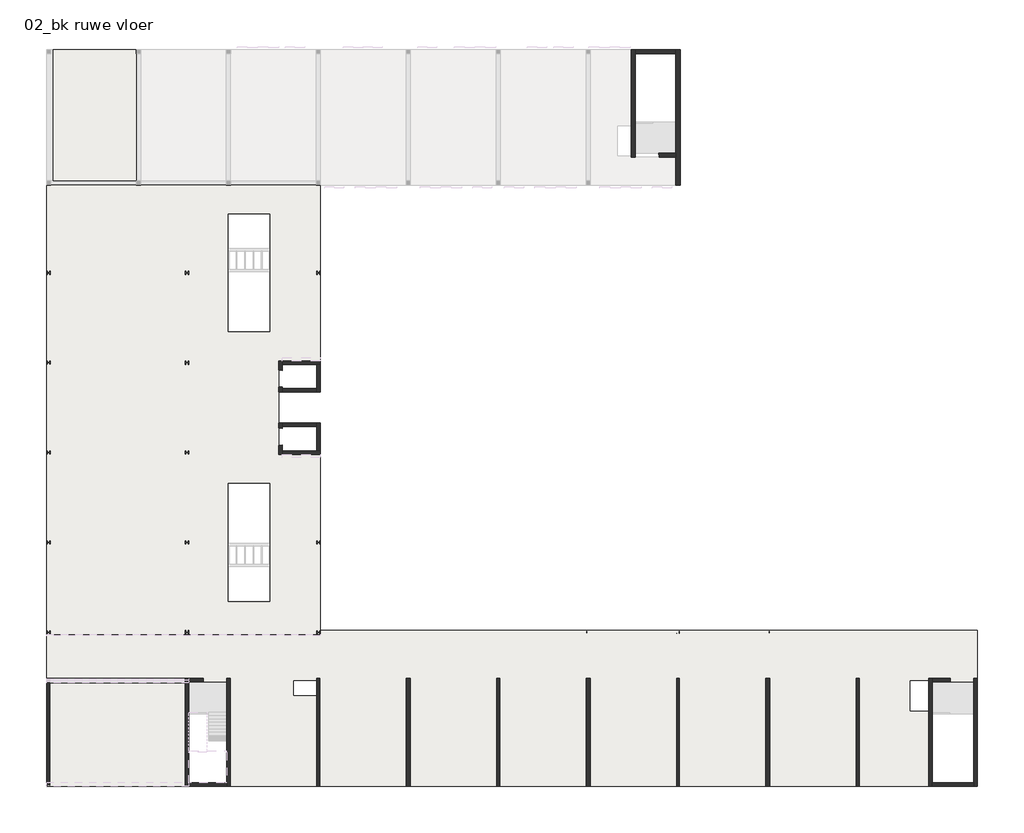
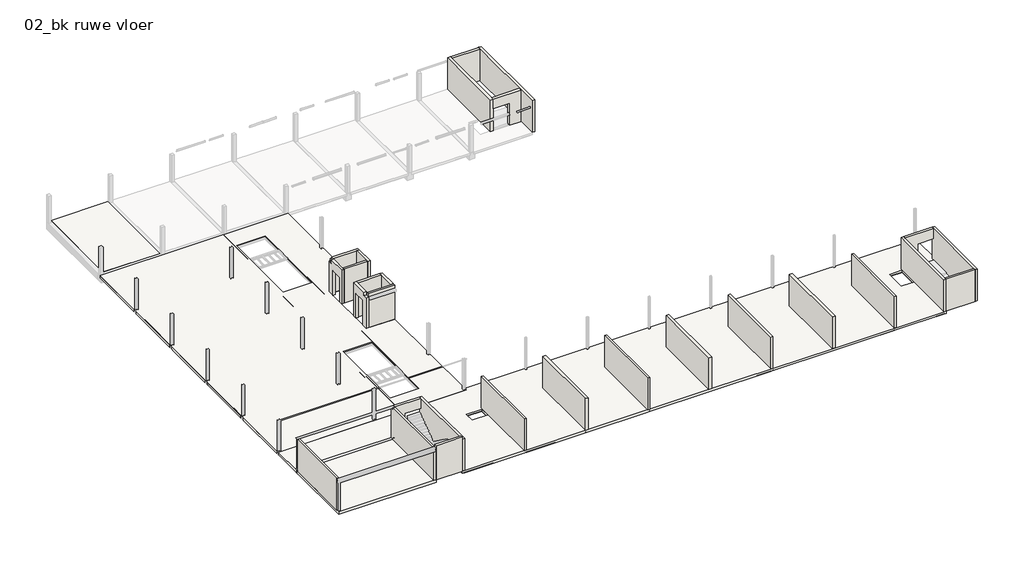
# One storey, part 1 of 3: 28 walls, 20 slabs.
# Revit data of these elements (continued)
# Element 16 (IfcSlab, "NLRS_23_FL_kanaalplaat 260_gen_rsf") (continued)
#   IfcGUID = "13lTCcCQ95UOWcvnmPh7yS"
#   built-in parameter 1001955 = 1.5708 (stored number, unit not read)
#   Height Offset From Level = -70 mm
#   built-in parameter 1001954 = 1
#   IsExternal = no
#   LoadBearing = yes
#   Phase Created = NLRS_nieuw
#   Materials on its faces: "NLRS_f2_beton prefab_gen_rsf"
# Element 17 (IfcSlab, "NLRS_23_FL_breedplaat 260_gen_rsf")
#   IfcGUID = "3aMdMHoe12P9KDGPyaIhfl"
#   built-in parameter 1001955 = 1.5708 (stored number, unit not read)
#   Height Offset From Level = 0 mm
#   built-in parameter 1001954 = 1
#   IsExternal = no
#   LoadBearing = yes
#   Phase Created = NLRS_nieuw
#   Materials on its faces: "NLRS_f2_beton ihwg_gen_rsf"
# Element 18 (IfcSlab, "NLRS_23_FL_breedplaat schil 60_gen_rsf")
#   IfcGUID = "30fJl_yZvFzewSfsmFGxtY"
#   Comments = ""
#   Height Offset From Level = -200 mm
#   built-in parameter 1001954 = 1
#   IsExternal = no
#   LoadBearing = yes
#   Phase Created = NLRS_nieuw
#   Materials on its faces: "NLRS_f2_beton prefab_gen_rsf"
# Element 19 (IfcSlab, "NLRS_23_FL_breedplaat schil 60_gen_rsf")
#   IfcGUID = "2NjBJrSTnArAq_EA_3B3B5"
#   Comments = ""
#   built-in parameter 1001955 = -1.5708 (stored number, unit not read)
#   Height Offset From Level = -200 mm
#   built-in parameter 1001954 = 1
#   IsExternal = no
#   LoadBearing = yes
#   Phase Created = NLRS_nieuw
#   Materials on its faces: "NLRS_f2_beton prefab_gen_rsf"
# Element 20 (IfcSlab, "NLRS_23_FL_breedplaat schil 60_gen_rsf")
#   IfcGUID = "2qE$kEBNbDT8O3EB3ypEdt"
#   Comments = ""
#   Height Offset From Level = -200 mm
#   built-in parameter 1001954 = 1
#   IsExternal = no
#   LoadBearing = yes
#   Phase Created = NLRS_nieuw
#   Materials on its faces: "NLRS_f2_beton prefab_gen_rsf"
# Element 21 (IfcWall, "NLRS_22_WA_beton ihw 250_gen_rsf")
#   IfcGUID = "13lTCcCQ95UOWcvnmPh77b"
#   Comments = ""
#   Top Offset = 0 mm
#   Base Offset = 0 mm
#   wall height = 3540 mm
#   IsExternal = no
#   LoadBearing = yes
#   Phase Created = NLRS_nieuw
#   Base Constraint = 02_bk ruwe vloer
#   Top Constraint = 03_ok ruwe vloer
#   Materials on its faces: "NLRS_f2_beton ihwg_gen_rsf"
# Element 22 (IfcWall, "NLRS_22_WA_beton ihw 250_gen_rsf")
#   IfcGUID = "13lTCcCQ95UOWcvnmPh77d"
#   Comments = ""
#   Top Offset = 0 mm
#   Base Offset = 0 mm
#   wall height = 3540 mm
#   IsExternal = no
#   LoadBearing = yes
#   Phase Created = NLRS_nieuw
#   Base Constraint = 02_bk ruwe vloer
#   Top Constraint = 03_ok ruwe vloer
#   Materials on its faces: "NLRS_f2_beton ihwg_gen_rsf"
# Element 23 (IfcWall, "NLRS_22_WA_kalkzandsteen CS12 214_gen_rsf")
#   IfcGUID = "13lTCcCQ95UOWcvnmPh77X"
#   Comments = ""
#   Top Offset = 0 mm
#   Base Offset = 0 mm
#   wall height = 3540 mm
#   IsExternal = no
#   LoadBearing = yes
#   Phase Created = NLRS_nieuw
#   Base Constraint = 02_bk ruwe vloer
#   Top Constraint = 03_ok ruwe vloer
#   Materials on its faces: "NLRS_f1_kalkzandsteen_gen_rsf"
# Element 24 (IfcWall, "NLRS_22_WA_beton ihw 300_gen_rsf")
#   IfcGUID = "13lTCcCQ95UOWcvnmPh77Z"
#   Comments = ""
#   Top Offset = 0 mm
#   Base Offset = 0 mm
#   wall height = 3540 mm
#   IsExternal = no
#   LoadBearing = yes
#   Phase Created = NLRS_nieuw
#   Base Constraint = 02_bk ruwe vloer
#   Top Constraint = 03_ok ruwe vloer
#   Materials on its faces: "NLRS_f2_beton ihwg_gen_rsf"
# Element 25 (IfcWall, "NLRS_22_WA_kalkzandsteen CS12 214_gen_rsf")
#   IfcGUID = "13lTCcCQ95UOWcvnmPh78T"
#   Comments = ""
#   Top Offset = 0 mm
#   Base Offset = 0 mm
#   wall height = 3540 mm
#   IsExternal = no
#   LoadBearing = yes
#   Phase Created = NLRS_nieuw
#   Base Constraint = 02_bk ruwe vloer
#   Top Constraint = 03_ok ruwe vloer
#   Materials on its faces: "NLRS_f1_kalkzandsteen_gen_rsf"
# Element 26 (IfcWall, "NLRS_22_WA_beton ihw 300_gen_rsf")
#   IfcGUID = "13lTCcCQ95UOWcvnmPh78V"
#   Comments = ""
#   Top Offset = 0 mm
#   Base Offset = 0 mm
#   wall height = 3540 mm
#   IsExternal = no
#   LoadBearing = yes
#   Phase Created = NLRS_nieuw
#   Base Constraint = 02_bk ruwe vloer
#   Top Constraint = 03_ok ruwe vloer
#   Materials on its faces: "NLRS_f2_beton ihwg_gen_rsf"
# Element 27 (IfcWall, "NLRS_22_WA_kalkzandsteen CS12 214_gen_rsf")
#   IfcGUID = "13lTCcCQ95UOWcvnmPh78P"
#   Comments = ""
#   Top Offset = 0 mm
#   Base Offset = 0 mm
#   wall height = 3540 mm
#   IsExternal = no
#   LoadBearing = yes
#   Phase Created = NLRS_nieuw
#   Base Constraint = 02_bk ruwe vloer
#   Top Constraint = 03_ok ruwe vloer
#   Materials on its faces: "NLRS_f1_kalkzandsteen_gen_rsf"
# Element 28 (IfcWall, "NLRS_22_WA_beton ihw 300_gen_rsf")
#   IfcGUID = "13lTCcCQ95UOWcvnmPh78R"
#   Comments = ""
#   Top Offset = 0 mm
#   Base Offset = 0 mm
#   wall height = 3540 mm
#   IsExternal = no
#   LoadBearing = yes
#   Phase Created = NLRS_nieuw
#   Base Constraint = 02_bk ruwe vloer
#   Top Constraint = 03_ok ruwe vloer
#   Materials on its faces: "NLRS_f2_beton ihwg_gen_rsf"
# Element 29 (IfcWall, "NLRS_22_WA_kalkzandsteen CS12 214_gen_rsf")
#   IfcGUID = "13lTCcCQ95UOWcvnmPh78L"
#   Comments = ""
#   Top Offset = 0 mm
#   Base Offset = 0 mm
#   wall height = 3540 mm
#   IsExternal = no
#   LoadBearing = yes
#   Phase Created = NLRS_nieuw
#   Base Constraint = 02_bk ruwe vloer
#   Top Constraint = 03_ok ruwe vloer
#   Materials on its faces: "NLRS_f1_kalkzandsteen_gen_rsf"
# Element 30 (IfcWall, "NLRS_21_WA_beton ihw 250_gen_rsf")
#   IfcGUID = "13lTCcCQ95UOWcvnmPh78N"
#   Comments = ""
#   Top Offset = 0 mm
#   Base Offset = 0 mm
#   wall height = 3540 mm
#   IsExternal = yes
#   LoadBearing = yes
#   Phase Created = NLRS_nieuw
#   Base Constraint = 02_bk ruwe vloer
#   Top Constraint = 03_ok ruwe vloer
#   Materials on its faces: "NLRS_f2_beton ihwg_gen_rsf"
# Element 31 (IfcWall, "NLRS_21_WA_kalkzandsteen CS12 214_gen_rsf")
#   IfcGUID = "13lTCcCQ95UOWcvnmPh78H"
#   Comments = ""
#   Top Offset = 0 mm
#   Base Offset = 0 mm
#   wall height = 3540 mm
#   IsExternal = yes
#   LoadBearing = yes
#   Phase Created = NLRS_nieuw
#   Base Constraint = 02_bk ruwe vloer
#   Top Constraint = 03_ok ruwe vloer
#   Materials on its faces: "NLRS_f1_kalkzandsteen_gen_rsf"
# Element 32 (IfcWall, "NLRS_21_WA_beton ihw 250_gen_rsf")
#   IfcGUID = "13lTCcCQ95UOWcvnmPh78J"
#   Top Offset = 0 mm
#   Base Offset = 0 mm
#   wall height = 3800 mm
#   IsExternal = yes
#   LoadBearing = yes
#   Phase Created = NLRS_nieuw
#   Base Constraint = 02_bk ruwe vloer
#   Top Constraint = 03_bk. ruwe vloer
#   Materials on its faces: "NLRS_f2_beton ihwg_gen_rsf"
# Element 33 (IfcWall, "NLRS_22_WA_beton ihw 250_gen_rsf")
#   IfcGUID = "13lTCcCQ95UOWcvnmPh78D"
#   Top Offset = 0 mm
#   Base Offset = 0 mm
#   wall height = 3540 mm
#   IsExternal = no
#   LoadBearing = yes
#   Phase Created = NLRS_nieuw
#   Base Constraint = 02_bk ruwe vloer
#   Top Constraint = 03_ok ruwe vloer
#   Materials on its faces: "NLRS_f2_beton ihwg_gen_rsf"
# Element 34 (IfcWall, "NLRS_22_WA_beton ihw 250_gen_rsf")
#   IfcGUID = "13lTCcCQ95UOWcvnmPh78F"
#   Comments = ""
#   Top Offset = 0 mm
#   Base Offset = 0 mm
#   wall height = 3540 mm
#   IsExternal = no
#   LoadBearing = yes
#   Phase Created = NLRS_nieuw
#   Base Constraint = 02_bk ruwe vloer
#   Top Constraint = 03_ok ruwe vloer
#   Materials on its faces: "NLRS_f2_beton ihwg_gen_rsf"
# Element 35 (IfcWall, "NLRS_21_WA_beton ihw 250_gen_rsf")
#   IfcGUID = "13lTCcCQ95UOWcvnmPh789"
#   Top Offset = 0 mm
#   Base Offset = 0 mm
#   wall height = 3540 mm
#   IsExternal = yes
#   LoadBearing = yes
#   Phase Created = NLRS_nieuw
#   Base Constraint = 02_bk ruwe vloer
#   Top Constraint = 03_ok ruwe vloer
#   Materials on its faces: "NLRS_f2_beton ihwg_gen_rsf"
# Element 36 (IfcWall, "NLRS_22_WA_beton ihw 250_gen_rsf")
#   IfcGUID = "13lTCcCQ95UOWcvnmPh78B"
#   Top Offset = 0 mm
#   Base Offset = 0 mm
#   wall height = 3540 mm
#   IsExternal = no
#   LoadBearing = yes
#   Phase Created = NLRS_nieuw
#   Base Constraint = 02_bk ruwe vloer
#   Top Constraint = 03_ok ruwe vloer
#   Materials on its faces: "NLRS_f2_beton ihwg_gen_rsf"
# Element 37 (IfcWall, "NLRS_22_WA_beton prefab 300_gen_rsf")
#   IfcGUID = "13lTCcCQ95UOWcvnmPh79n"
#   Comments = ""
#   built-in parameter 1001111 = 20 mm
#   Top Offset = 0 mm
#   Base Offset = 20 mm
#   wall height = 3520 mm
#   IsExternal = no
#   LoadBearing = yes
#   Phase Created = NLRS_nieuw
#   Base Constraint = 02_bk ruwe vloer
#   Top Constraint = 03_ok ruwe vloer
#   Materials on its faces: "NLRS_f2_beton prefab_gen_rsf"
# Element 38 (IfcWall, "NLRS_21_WA_beton prefab 300_gen_rsf")
#   IfcGUID = "13lTCcCQ95UOWcvnmPh79k"
#   Comments = ""
#   built-in parameter 1001111 = 20 mm
#   Top Offset = 0 mm
#   Base Offset = 20 mm
#   wall height = 3520 mm
#   IsExternal = yes
#   LoadBearing = yes
#   Phase Created = NLRS_nieuw
#   Base Constraint = 02_bk ruwe vloer
#   Top Constraint = 03_ok ruwe vloer
#   Materials on its faces: "NLRS_f2_beton prefab_gen_rsf"
# Element 39 (IfcWall, "NLRS_21_WA_beton prefab 300_gen_rsf")
#   IfcGUID = "13lTCcCQ95UOWcvnmPh79e"
#   Comments = ""
#   built-in parameter 1001111 = 20 mm
#   Top Offset = 0 mm
#   Base Offset = 20 mm
#   wall height = 3520 mm
#   IsExternal = yes
#   LoadBearing = yes
#   Phase Created = NLRS_nieuw
#   Base Constraint = 02_bk ruwe vloer
#   Top Constraint = 03_ok ruwe vloer
#   Materials on its faces: "NLRS_f2_beton prefab_gen_rsf"
# Element 40 (IfcWall, "NLRS_22_WA_beton prefab 300_gen_rsf")
#   IfcGUID = "13lTCcCQ95UOWcvnmPh79g"
#   Comments = ""
#   built-in parameter 1001111 = 20 mm
#   Top Offset = 0 mm
#   Base Offset = 20 mm
#   wall height = 3520 mm
#   IsExternal = no
#   LoadBearing = yes
#   Phase Created = NLRS_nieuw
#   Base Constraint = 02_bk ruwe vloer
#   Top Constraint = 03_ok ruwe vloer
#   Materials on its faces: "NLRS_f2_beton prefab_gen_rsf"
# Element 41 (IfcWall, "NLRS_22_WA_beton prefab 250_gen_rsf")
#   IfcGUID = "13lTCcCQ95UOWcvnmPh7B5"
#   built-in parameter 1001111 = 20 mm
#   Top Offset = 0 mm
#   Base Offset = 20 mm
#   wall height = 3780 mm
#   IsExternal = no
#   LoadBearing = yes
#   Phase Created = NLRS_nieuw
#   Base Constraint = 02_bk ruwe vloer
#   Top Constraint = 03_bk. ruwe vloer
#   Materials on its faces: "NLRS_f2_beton prefab_gen_rsf"
# Element 42 (IfcWall, "NLRS_22_WA_beton prefab 250_gen_rsf")
#   IfcGUID = "13lTCcCQ95UOWcvnmPh7B7"
#   built-in parameter 1001111 = 20 mm
#   Top Offset = 0 mm
#   Base Offset = 20 mm
#   wall height = 3780 mm
#   IsExternal = no
#   LoadBearing = yes
#   Phase Created = NLRS_nieuw
#   Base Constraint = 02_bk ruwe vloer
#   Top Constraint = 03_bk. ruwe vloer
#   Materials on its faces: "NLRS_f2_beton prefab_gen_rsf"
# Element 43 (IfcWall, "NLRS_22_WA_beton prefab 250_gen_rsf")
#   IfcGUID = "13lTCcCQ95UOWcvnmPh7B1"
#   built-in parameter 1001111 = 20 mm
#   Top Offset = 0 mm
#   Base Offset = 20 mm
#   wall height = 3780 mm
#   IsExternal = no
#   LoadBearing = yes
#   Phase Created = NLRS_nieuw
#   Base Constraint = 02_bk ruwe vloer
#   Top Constraint = 03_bk. ruwe vloer
#   Materials on its faces: "NLRS_f2_beton prefab_gen_rsf"
# Element 44 (IfcWall, "NLRS_21_WA_beton prefab 250_gen_rsf")
#   IfcGUID = "13lTCcCQ95UOWcvnmPh7B3"
#   built-in parameter 1001111 = 20 mm
#   Top Offset = 0 mm
#   Base Offset = 20 mm
#   wall height = 3780 mm
#   IsExternal = yes
#   LoadBearing = yes
#   Phase Created = NLRS_nieuw
#   Base Constraint = 02_bk ruwe vloer
#   Top Constraint = 03_bk. ruwe vloer
#   Materials on its faces: "NLRS_f2_beton prefab_gen_rsf"
# Element 45 (IfcWall, "NLRS_22_WA_beton prefab 250_gen_rsf")
#   IfcGUID = "13lTCcCQ95UOWcvnmPh7Bz"
#   built-in parameter 1001111 = 20 mm
#   Top Offset = 0 mm
#   Base Offset = 20 mm
#   wall height = 3780 mm
#   IsExternal = no
#   LoadBearing = yes
#   Phase Created = NLRS_nieuw
#   Base Constraint = 02_bk ruwe vloer
#   Top Constraint = 03_bk. ruwe vloer
#   Materials on its faces: "NLRS_f2_beton prefab_gen_rsf"
# Element 46 (IfcWall, "NLRS_22_WA_beton prefab 250_gen_rsf")
#   IfcGUID = "13lTCcCQ95UOWcvnmPh7B$"
#   built-in parameter 1001111 = 20 mm
#   Top Offset = 0 mm
#   Base Offset = 20 mm
#   wall height = 3780 mm
#   IsExternal = no
#   LoadBearing = yes
#   Phase Created = NLRS_nieuw
#   Base Constraint = 02_bk ruwe vloer
#   Top Constraint = 03_bk. ruwe vloer
#   Materials on its faces: "NLRS_f2_beton prefab_gen_rsf"
# Element 47 (IfcWall, "NLRS_22_WA_beton prefab 250_gen_rsf")
#   IfcGUID = "13lTCcCQ95UOWcvnmPh7Bv"
#   built-in parameter 1001111 = 20 mm
#   Top Offset = 0 mm
#   Base Offset = 20 mm
#   wall height = 3780 mm
#   IsExternal = no
#   LoadBearing = yes
#   Phase Created = NLRS_nieuw
#   Base Constraint = 02_bk ruwe vloer
#   Top Constraint = 03_bk. ruwe vloer
#   Materials on its faces: "NLRS_f2_beton prefab_gen_rsf"
# Element 48 (IfcWall, "NLRS_21_WA_beton prefab 250_gen_rsf")
#   IfcGUID = "13lTCcCQ95UOWcvnmPh7Bx"
#   built-in parameter 1001111 = 20 mm
#   Top Offset = 0 mm
#   Base Offset = 20 mm
#   wall height = 3780 mm
#   IsExternal = yes
#   LoadBearing = yes
#   Phase Created = NLRS_nieuw
#   Base Constraint = 02_bk ruwe vloer
#   Top Constraint = 03_bk. ruwe vloer
#   Materials on its faces: "NLRS_f2_beton prefab_gen_rsf"
# Materials
#   "NLRS_f2_beton ihwg_gen_rsf": class "F - Niet gebakken kunststeen", colour RGB 129 133 118, transparency 0, Keynote = "f2", Manufacturer = "Revit Standards Foundation", URL = "www.revitstandards.org", Description = "beton ihwg", Cost = 0
#   "NLRS_f2_beton prefab_gen_rsf": class "F - Niet gebakken kunststeen", colour RGB 129 133 118, transparency 0, Keynote = "f2", Manufacturer = "Revit Standards Foundation", URL = "www.revitstandards.org", Description = "beton prefab", Cost = 0
#   "NLRS_f1_kalkzandsteen_gen_rsf": class "F - Niet gebakken kunststeen", colour RGB 223 221 219, transparency 0, Keynote = "f1", Manufacturer = "Revit Standards Foundation", URL = "www.revitstandards.org", Description = "kalkzandsteen", Cost = 0
